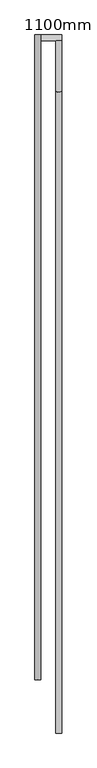
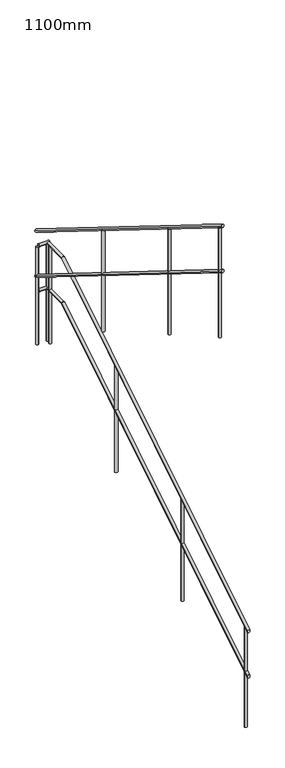
"""IFC4 building model written with IfcOpenShell, lengths in millimetres: railing geometry, 1100mm."""

from ifc_helpers import new_model, si_unit, point, frame, frame_2d, origin, place, context, project, spatial, circle_curve, ellipse_curve, trimmed, segment, composite_curve, outline, extrude, source, transform, mapped, element, save
from ifc_brep_helpers import plane_surface, cylinder_surface, advanced_brep


def railing_1100mm_1ac2519f(model_context):
    return source(origin(), model_context, "Body", "SolidModel", [
        advanced_brep(
        [(11545.1052251, 14699.5208589, 456.3396197), (11515.1052251, 14699.5208589, 456.3396197), (11545.1052251, 18329.5208589, 2547.0), (11515.1052251, 18329.5208589, 2547.0), (11545.1052251, 18063.8019306, 2547.0), (11515.1052251, 18063.8019306, 2547.0)],
        [
            (0, 1, ellipse_curve(frame((11530.1052251, 14699.5208589, 456.3396197), z_axis=(0.0, -1.0, 0.0), x_axis=(0.0, 0.0, -1.0)), 17.6603803, 15.0)),
            (1, 0, ellipse_curve(frame((11530.1052251, 14699.5208589, 456.3396197), z_axis=(0.0, -1.0, 0.0), x_axis=(0.0, 0.0, -1.0)), 17.6603803, 15.0)),
            (2, 3, circle_curve(frame((11530.1052251, 18329.5208589, 2547.0), z_axis=(0.0, 1.0, 0.0), x_axis=(-1.0, 0.0, 0.0)), 15.0)),
            (3, 2, circle_curve(frame((11530.1052251, 18329.5208589, 2547.0), z_axis=(0.0, 1.0, 0.0), x_axis=(-1.0, 0.0, 0.0)), 15.0)),
            (0, 4),
            (4, 5, ellipse_curve(frame((11530.1052251, 18063.8019306, 2547.0), z_axis=(0.0, -0.9616025257983003, -0.2744459552959912), x_axis=(0.0, 0.2744459552959914, -0.9616025257983002)), 15.5989607, 15.0)),
            (5, 1),
            (5, 4, ellipse_curve(frame((11530.1052251, 18063.8019306, 2547.0), z_axis=(0.0, -0.9616025257983003, -0.2744459552959912), x_axis=(0.0, 0.2744459552959914, -0.9616025257983002)), 15.5989607, 15.0)),
            (4, 2),
            (3, 5),
        ],
        [
            plane_surface(frame((11530.1052251, 14699.5208589, 474.0), z_axis=(0.0, -1.0, 0.0), x_axis=(0.0, 0.0, 1.0))),
            plane_surface(frame((11530.1052251, 18329.5208589, 2562.0), z_axis=(0.0, 1.0, 0.0), x_axis=(0.0, 0.0, 1.0))),
            cylinder_surface(frame((11530.1052251, 14707.4380966, 461.2596175), z_axis=(0.0, -0.8493588352433417, -0.5278158476155052), x_axis=(-1.0, 0.0, 0.0)), 15.0),
            cylinder_surface(frame((11530.1052251, 18059.5208589, 2547.0), z_axis=(0.0, -1.0, 0.0), x_axis=(-1.0, 0.0, 0.0)), 15.0),
        ],
        [
            (0, [[1, 2]]),
            (1, [[3, 4]]),
            (2, [[-1, 5, 6, 7]]),
            (2, [[-2, -7, 8, -5]]),
            (3, [[-6, 9, -4, 10]]),
            (3, [[-8, -10, -3, -9]]),
        ],
    ),
        advanced_brep(
        [(11545.1052251, 18359.5208589, 2547.0), (11545.1052251, 18329.5208589, 2547.0), (11435.1052251, 18359.5208589, 2547.0), (11435.1052251, 18329.5208589, 2547.0)],
        [
            (0, 1, circle_curve(frame((11545.1052251, 18344.5208589, 2547.0), z_axis=(1.0, 0.0, 0.0), x_axis=(0.0, -1.0, 0.0)), 15.0)),
            (1, 0, circle_curve(frame((11545.1052251, 18344.5208589, 2547.0), z_axis=(1.0, 0.0, 0.0), x_axis=(0.0, -1.0, 0.0)), 15.0)),
            (2, 3, circle_curve(frame((11435.1052251, 18344.5208589, 2547.0), z_axis=(-1.0, 0.0, 0.0), x_axis=(0.0, -1.0, 0.0)), 15.0)),
            (3, 2, circle_curve(frame((11435.1052251, 18344.5208589, 2547.0), z_axis=(-1.0, 0.0, 0.0), x_axis=(0.0, -1.0, 0.0)), 15.0)),
            (0, 2),
            (3, 1),
        ],
        [
            plane_surface(frame((11545.1052251, 18344.5208589, 2562.0), z_axis=(1.0, 0.0, 0.0), x_axis=(0.0, -1.0, 0.0))),
            plane_surface(frame((11435.1052251, 18344.5208589, 2562.0), z_axis=(-1.0, 0.0, 0.0), x_axis=(0.0, -1.0, 0.0))),
            cylinder_surface(frame((11545.1052251, 18344.5208589, 2547.0), z_axis=(1.0, 0.0, 0.0), x_axis=(0.0, -1.0, 0.0)), 15.0),
        ],
        [
            (0, [[1, 2]]),
            (1, [[3, 4]]),
            (2, [[-1, 5, -4, 6]]),
            (2, [[-2, -6, -3, -5]]),
        ],
    ),
        advanced_brep(
        [(11405.1052251, 18359.5208589, 2705.9110483), (11435.1052251, 18359.5208589, 2705.9110483), (11405.1052251, 14979.5208589, 4806.3396197), (11435.1052251, 14979.5208589, 4806.3396197)],
        [
            (0, 1, ellipse_curve(frame((11420.1052251, 18359.5208589, 2705.9110483), z_axis=(0.0, 1.0, 0.0), x_axis=(0.0, 0.0, -1.0)), 17.6603803, 15.0)),
            (1, 0, ellipse_curve(frame((11420.1052251, 18359.5208589, 2705.9110483), z_axis=(0.0, 1.0, 0.0), x_axis=(0.0, 0.0, -1.0)), 17.6603803, 15.0)),
            (2, 3, ellipse_curve(frame((11420.1052251, 14979.5208589, 4806.3396197), z_axis=(0.0, -1.0, 0.0), x_axis=(0.0, 0.0, -1.0)), 17.6603803, 15.0)),
            (3, 2, ellipse_curve(frame((11420.1052251, 14979.5208589, 4806.3396197), z_axis=(0.0, -1.0, 0.0), x_axis=(0.0, 0.0, -1.0)), 17.6603803, 15.0)),
            (0, 2),
            (3, 1),
        ],
        [
            plane_surface(frame((11420.1052251, 18359.5208589, 2723.5714286), z_axis=(0.0, 1.0, 0.0), x_axis=(0.0, 0.0, -1.0))),
            plane_surface(frame((11420.1052251, 14979.5208589, 4824.0), z_axis=(0.0, -1.0, 0.0), x_axis=(0.0, 0.0, -1.0))),
            cylinder_surface(frame((11420.1052251, 18351.6036212, 2710.831046), z_axis=(0.0, 0.8493588352433417, -0.5278158476155052), x_axis=(1.0, 0.0, 0.0)), 15.0),
        ],
        [
            (0, [[1, 2]]),
            (1, [[3, 4]]),
            (2, [[-1, 5, -4, 6]]),
            (2, [[-2, -6, -3, -5]]),
        ],
    ),
        advanced_brep(
        [(11545.1052251, 14699.5208589, 956.3396197), (11515.1052251, 14699.5208589, 956.3396197), (11545.1052251, 18063.8019306, 3047.0), (11515.1052251, 18063.8019306, 3047.0), (11545.1052251, 18329.5208589, 3047.0), (11515.1052251, 18329.5208589, 3047.0)],
        [
            (0, 1, ellipse_curve(frame((11530.1052251, 14699.5208589, 956.3396197), z_axis=(0.0, -1.0, 0.0), x_axis=(0.0, 0.0, -1.0)), 17.6603803, 15.0)),
            (1, 0, ellipse_curve(frame((11530.1052251, 14699.5208589, 956.3396197), z_axis=(0.0, -1.0, 0.0), x_axis=(0.0, 0.0, -1.0)), 17.6603803, 15.0)),
            (0, 2),
            (2, 3, ellipse_curve(frame((11530.1052251, 18063.8019306, 3047.0), z_axis=(0.0, -0.9616025257983003, -0.2744459552959912), x_axis=(0.0, 0.2744459552959914, -0.9616025257983002)), 15.5989607, 15.0)),
            (3, 1),
            (3, 2, ellipse_curve(frame((11530.1052251, 18063.8019306, 3047.0), z_axis=(0.0, -0.9616025257983003, -0.2744459552959912), x_axis=(0.0, 0.2744459552959914, -0.9616025257983002)), 15.5989607, 15.0)),
            (4, 5, circle_curve(frame((11530.1052251, 18329.5208589, 3047.0), z_axis=(0.0, 1.0, 0.0), x_axis=(-1.0, 0.0, 0.0)), 15.0)),
            (5, 4, circle_curve(frame((11530.1052251, 18329.5208589, 3047.0), z_axis=(0.0, 1.0, 0.0), x_axis=(-1.0, 0.0, 0.0)), 15.0)),
            (2, 4),
            (5, 3),
        ],
        [
            plane_surface(frame((11530.1052251, 14699.5208589, 974.0), z_axis=(0.0, -1.0, 0.0), x_axis=(0.0, 0.0, 1.0))),
            cylinder_surface(frame((11530.1052251, 14707.4380966, 961.2596175), z_axis=(0.0, -0.8493588352433417, -0.5278158476155052), x_axis=(-1.0, 0.0, 0.0)), 15.0),
            plane_surface(frame((11530.1052251, 18329.5208589, 3062.0), z_axis=(0.0, 1.0, 0.0), x_axis=(0.0, 0.0, 1.0))),
            cylinder_surface(frame((11530.1052251, 18059.5208589, 3047.0), z_axis=(0.0, -1.0, 0.0), x_axis=(-1.0, 0.0, 0.0)), 15.0),
        ],
        [
            (0, [[1, 2]]),
            (1, [[-1, 3, 4, 5]]),
            (1, [[-2, -5, 6, -3]]),
            (2, [[7, 8]]),
            (3, [[-4, 9, -8, 10]]),
            (3, [[-6, -10, -7, -9]]),
        ],
    ),
        advanced_brep(
        [(11545.1052251, 18359.5208589, 3047.0), (11545.1052251, 18329.5208589, 3047.0), (11435.1052251, 18359.5208589, 3047.0), (11435.1052251, 18329.5208589, 3047.0)],
        [
            (0, 1, circle_curve(frame((11545.1052251, 18344.5208589, 3047.0), z_axis=(1.0, 0.0, 0.0), x_axis=(0.0, -1.0, 0.0)), 15.0)),
            (1, 0, circle_curve(frame((11545.1052251, 18344.5208589, 3047.0), z_axis=(1.0, 0.0, 0.0), x_axis=(0.0, -1.0, 0.0)), 15.0)),
            (2, 3, circle_curve(frame((11435.1052251, 18344.5208589, 3047.0), z_axis=(-1.0, 0.0, 0.0), x_axis=(0.0, -1.0, 0.0)), 15.0)),
            (3, 2, circle_curve(frame((11435.1052251, 18344.5208589, 3047.0), z_axis=(-1.0, 0.0, 0.0), x_axis=(0.0, -1.0, 0.0)), 15.0)),
            (0, 2),
            (3, 1),
        ],
        [
            plane_surface(frame((11545.1052251, 18344.5208589, 3062.0), z_axis=(1.0, 0.0, 0.0), x_axis=(0.0, -1.0, 0.0))),
            plane_surface(frame((11435.1052251, 18344.5208589, 3062.0), z_axis=(-1.0, 0.0, 0.0), x_axis=(0.0, -1.0, 0.0))),
            cylinder_surface(frame((11545.1052251, 18344.5208589, 3047.0), z_axis=(1.0, 0.0, 0.0), x_axis=(0.0, -1.0, 0.0)), 15.0),
        ],
        [
            (0, [[1, 2]]),
            (1, [[3, 4]]),
            (2, [[-1, 5, -4, 6]]),
            (2, [[-2, -6, -3, -5]]),
        ],
    ),
        advanced_brep(
        [(11405.1052251, 18359.5208589, 3205.9110483), (11435.1052251, 18359.5208589, 3205.9110483), (11405.1052251, 14979.5208589, 5306.3396197), (11435.1052251, 14979.5208589, 5306.3396197)],
        [
            (0, 1, ellipse_curve(frame((11420.1052251, 18359.5208589, 3205.9110483), z_axis=(0.0, 1.0, 0.0), x_axis=(0.0, 0.0, -1.0)), 17.6603803, 15.0)),
            (1, 0, ellipse_curve(frame((11420.1052251, 18359.5208589, 3205.9110483), z_axis=(0.0, 1.0, 0.0), x_axis=(0.0, 0.0, -1.0)), 17.6603803, 15.0)),
            (2, 3, ellipse_curve(frame((11420.1052251, 14979.5208589, 5306.3396197), z_axis=(0.0, -1.0, 0.0), x_axis=(0.0, 0.0, -1.0)), 17.6603803, 15.0)),
            (3, 2, ellipse_curve(frame((11420.1052251, 14979.5208589, 5306.3396197), z_axis=(0.0, -1.0, 0.0), x_axis=(0.0, 0.0, -1.0)), 17.6603803, 15.0)),
            (0, 2),
            (3, 1),
        ],
        [
            plane_surface(frame((11420.1052251, 18359.5208589, 3223.5714286), z_axis=(0.0, 1.0, 0.0), x_axis=(0.0, 0.0, -1.0))),
            plane_surface(frame((11420.1052251, 14979.5208589, 5324.0), z_axis=(0.0, -1.0, 0.0), x_axis=(0.0, 0.0, -1.0))),
            cylinder_surface(frame((11420.1052251, 18351.6036212, 3210.831046), z_axis=(0.0, 0.8493588352433417, -0.5278158476155052), x_axis=(1.0, 0.0, 0.0)), 15.0),
        ],
        [
            (0, [[1, 2]]),
            (1, [[3, 4]]),
            (2, [[-1, 5, -4, 6]]),
            (2, [[-2, -6, -3, -5]]),
        ],
    ),
        extrude(outline(composite_curve([segment(trimmed(circle_curve(frame_2d((11420.1052251, 15944.5208589)), 15.0), [point((11435.1052251, 15944.5208589))], [point((11405.1052251, 15944.5208589))], False, "CARTESIAN"), True, "CONTINUOUS"), segment(trimmed(circle_curve(frame_2d((11420.1052251, 15944.5208589)), 15.0), [point((11405.1052251, 15944.5208589))], [point((11435.1052251, 15944.5208589))], False, "CARTESIAN"), True, "CONTINUOUS")], self_intersect=False)), frame((0.0, 0.0, 3528.0), z_axis=(0.0, 0.0, 1.0), x_axis=(1.0, 0.0, 0.0)), (0.0, 0.0, 1.0), 1166.3214286),
        extrude(outline(composite_curve([segment(trimmed(circle_curve(frame_2d((11420.1052251, 17144.5208589)), 15.0), [point((11435.1052251, 17144.5208589))], [point((11405.1052251, 17144.5208589))], False, "CARTESIAN"), True, "CONTINUOUS"), segment(trimmed(circle_curve(frame_2d((11420.1052251, 17144.5208589)), 15.0), [point((11405.1052251, 17144.5208589))], [point((11435.1052251, 17144.5208589))], False, "CARTESIAN"), True, "CONTINUOUS")], self_intersect=False)), frame((0.0, 0.0, 2832.0), z_axis=(0.0, 0.0, 1.0), x_axis=(1.0, 0.0, 0.0)), (0.0, 0.0, 1.0), 1116.6071429),
        extrude(outline(composite_curve([segment(trimmed(circle_curve(frame_2d((11530.1052251, 18299.5208589)), 15.0), [point((11515.1052251, 18299.5208589))], [point((11545.1052251, 18299.5208589))], False, "CARTESIAN"), True, "CONTINUOUS"), segment(trimmed(circle_curve(frame_2d((11530.1052251, 18299.5208589)), 15.0), [point((11545.1052251, 18299.5208589))], [point((11515.1052251, 18299.5208589))], False, "CARTESIAN"), True, "CONTINUOUS")], self_intersect=False)), frame((0.0, 0.0, 1962.0), z_axis=(0.0, 0.0, 1.0), x_axis=(1.0, 0.0, 0.0)), (0.0, 0.0, 1.0), 1070.0),
        extrude(outline(composite_curve([segment(trimmed(circle_curve(frame_2d((11530.1052251, 17099.5208589)), 15.0), [point((11515.1052251, 17099.5208589))], [point((11545.1052251, 17099.5208589))], False, "CARTESIAN"), True, "CONTINUOUS"), segment(trimmed(circle_curve(frame_2d((11530.1052251, 17099.5208589)), 15.0), [point((11545.1052251, 17099.5208589))], [point((11515.1052251, 17099.5208589))], False, "CARTESIAN"), True, "CONTINUOUS")], self_intersect=False)), frame((0.0, 0.0, 1266.0), z_axis=(0.0, 0.0, 1.0), x_axis=(1.0, 0.0, 0.0)), (0.0, 0.0, 1.0), 1169.4285714),
        extrude(outline(composite_curve([segment(trimmed(circle_curve(frame_2d((11530.1052251, 15899.5208589)), 15.0), [point((11515.1052251, 15899.5208589))], [point((11545.1052251, 15899.5208589))], False, "CARTESIAN"), True, "CONTINUOUS"), segment(trimmed(circle_curve(frame_2d((11530.1052251, 15899.5208589)), 15.0), [point((11545.1052251, 15899.5208589))], [point((11515.1052251, 15899.5208589))], False, "CARTESIAN"), True, "CONTINUOUS")], self_intersect=False)), frame((0.0, 0.0, 570.0), z_axis=(0.0, 0.0, 1.0), x_axis=(1.0, 0.0, 0.0)), (0.0, 0.0, 1.0), 1119.7142857),
        extrude(outline(composite_curve([segment(trimmed(circle_curve(frame_2d((11420.1052251, 18344.5208589)), 15.0), [point((11420.1052251, 18329.5208589))], [point((11420.1052251, 18359.5208589))], False, "CARTESIAN"), True, "CONTINUOUS"), segment(trimmed(circle_curve(frame_2d((11420.1052251, 18344.5208589)), 15.0), [point((11420.1052251, 18359.5208589))], [point((11420.1052251, 18329.5208589))], False, "CARTESIAN"), True, "CONTINUOUS")], self_intersect=False)), frame((0.0, 0.0, 1962.0), z_axis=(0.0, 0.0, 1.0), x_axis=(1.0, 0.0, 0.0)), (0.0, 0.0, 1.0), 1070.0),
        extrude(outline(composite_curve([segment(trimmed(circle_curve(frame_2d((11530.1052251, 18344.5208589)), 15.0), [point((11515.1052251, 18344.5208589))], [point((11545.1052251, 18344.5208589))], False, "CARTESIAN"), True, "CONTINUOUS"), segment(trimmed(circle_curve(frame_2d((11530.1052251, 18344.5208589)), 15.0), [point((11545.1052251, 18344.5208589))], [point((11515.1052251, 18344.5208589))], False, "CARTESIAN"), True, "CONTINUOUS")], self_intersect=False)), frame((0.0, 0.0, 1962.0), z_axis=(0.0, 0.0, 1.0), x_axis=(1.0, 0.0, 0.0)), (0.0, 0.0, 1.0), 1070.0),
        extrude(outline(composite_curve([segment(trimmed(circle_curve(frame_2d((11420.1052251, 15029.5208589)), 15.0), [point((11435.1052251, 15029.5208589))], [point((11405.1052251, 15029.5208589))], False, "CARTESIAN"), True, "CONTINUOUS"), segment(trimmed(circle_curve(frame_2d((11420.1052251, 15029.5208589)), 15.0), [point((11405.1052251, 15029.5208589))], [point((11435.1052251, 15029.5208589))], False, "CARTESIAN"), True, "CONTINUOUS")], self_intersect=False)), frame((0.0, 0.0, 4050.0), z_axis=(0.0, 0.0, 1.0), x_axis=(1.0, 0.0, 0.0)), (0.0, 0.0, 1.0), 1212.9285714),
        extrude(outline(composite_curve([segment(trimmed(circle_curve(frame_2d((11530.1052251, 14749.5208589)), 15.0), [point((11515.1052251, 14749.5208589))], [point((11545.1052251, 14749.5208589))], False, "CARTESIAN"), True, "CONTINUOUS"), segment(trimmed(circle_curve(frame_2d((11530.1052251, 14749.5208589)), 15.0), [point((11545.1052251, 14749.5208589))], [point((11515.1052251, 14749.5208589))], False, "CARTESIAN"), True, "CONTINUOUS")], self_intersect=False)), frame((0.0, 0.0, -126.0), z_axis=(0.0, 0.0, 1.0), x_axis=(1.0, 0.0, 0.0)), (0.0, 0.0, 1.0), 1101.0714286),
    ])


if __name__ == "__main__":
    model = new_model("IFC4")
    model_context = context("Model", 3, world=origin())
    ifc_project = project(units=[si_unit("LENGTHUNIT", "METRE", prefix="MILLI")], contexts=[model_context])
    site = spatial("IfcSite", under=ifc_project)
    building = spatial("IfcBuilding", under=site)
    placement = place(None, origin())
    railing_1100mm_shape = railing_1100mm_1ac2519f(model_context)
    element("IfcRailing", 1, ObjectType="1100mm", at=placement, inside=building, context=model_context, shape_type="MappedRepresentation", body=[
        mapped(railing_1100mm_shape, transform((0.0, 0.0, 0.0), x_axis=(1.0, 0.0, 0.0), y_axis=(0.0, 1.0, 0.0), z_axis=(0.0, 0.0, 1.0))),
    ])
    save(model, "model.ifc")
